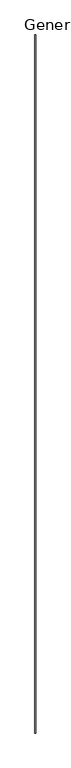
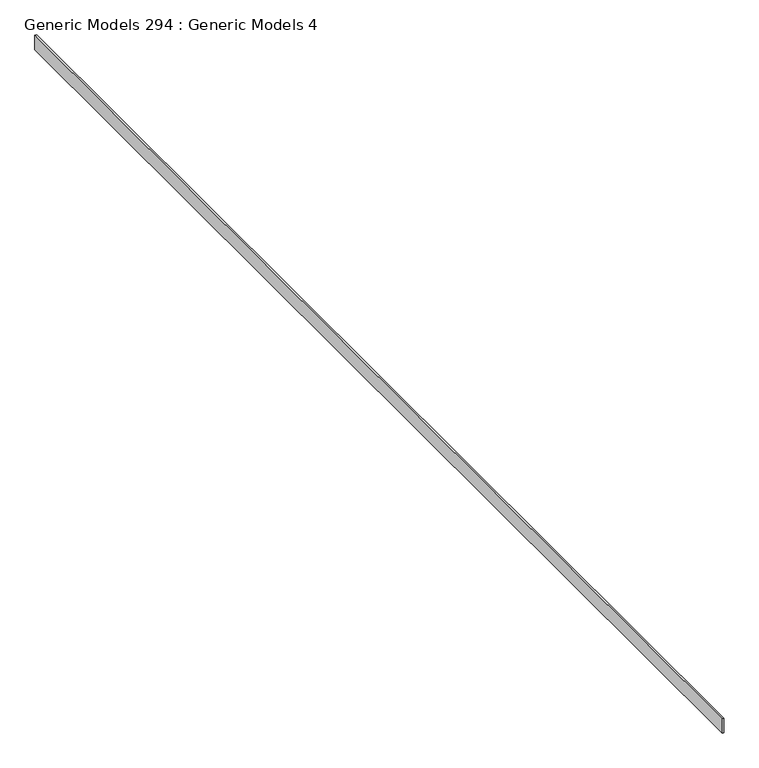
"""IFC4 building model written with IfcOpenShell, lengths in millimetres: proxy geometry, Generic Models 294 : Generic Models 4."""

from ifc_helpers import new_model, si_unit, frame, origin, place, context, project, spatial, polyline, outline, extrude, source, transform, mapped, element, save


def generic_models_294_generic_models_4_2e7edc5e(model_context):
    return source(origin(), model_context, "Body", "SweptSolid", [
        extrude(outline(polyline([(-7055.3152497, -6864.9230338), (-7064.4438133, -6864.9230338), (-7064.4438133, -464.1230338), (-7055.3152497, -464.1230338), (-7055.3152497, -6864.9230338)])), frame((0.0, 0.0, 127253.746), z_axis=(0.0, 0.0, 1.0), x_axis=(1.0, 0.0, 0.0)), (0.0, 0.0, 1.0), 81.0276561),
    ])


if __name__ == "__main__":
    model = new_model("IFC4")
    model_context = context("Model", 3, world=origin())
    ifc_project = project(units=[si_unit("LENGTHUNIT", "METRE", prefix="MILLI")], contexts=[model_context])
    site = spatial("IfcSite", under=ifc_project)
    building = spatial("IfcBuilding", under=site)
    placement = place(None, origin())
    generic_models_294_generic_models_4_shape = generic_models_294_generic_models_4_2e7edc5e(model_context)
    element("IfcBuildingElementProxy", 1, Name="Generic Models 294 : Generic Models 4", ObjectType="Generic Models 294 : Generic Models 4", at=placement, inside=building, context=model_context, shape_type="MappedRepresentation", body=[
        mapped(generic_models_294_generic_models_4_shape, transform((0.0, 0.0, 0.0), x_axis=(1.0, 0.0, 0.0), y_axis=(0.0, 1.0, 0.0), z_axis=(0.0, 0.0, 1.0))),
    ])
    save(model, "model.ifc")

# Revit data of these elements
# Element 1 (IfcBuildingElementProxy, "Generic Models 294 : Generic Models 4")
#   Materials on its faces: "_BLOCKING AS REQUIRED"
# Materials
#   "_BLOCKING AS REQUIRED": class "Generic", colour RGB 177 130 114, transparency 0, Cost = 0
